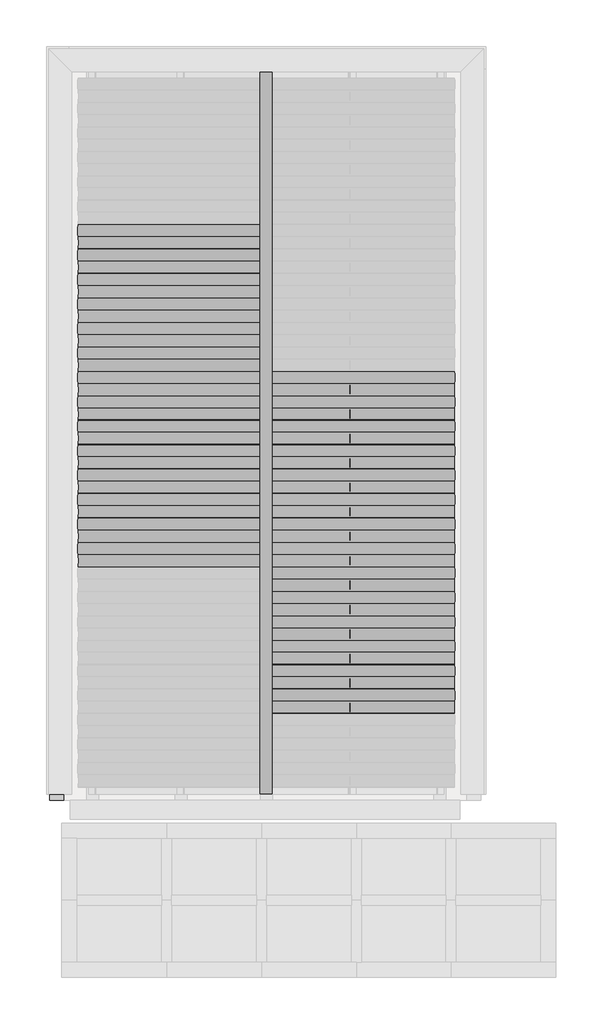
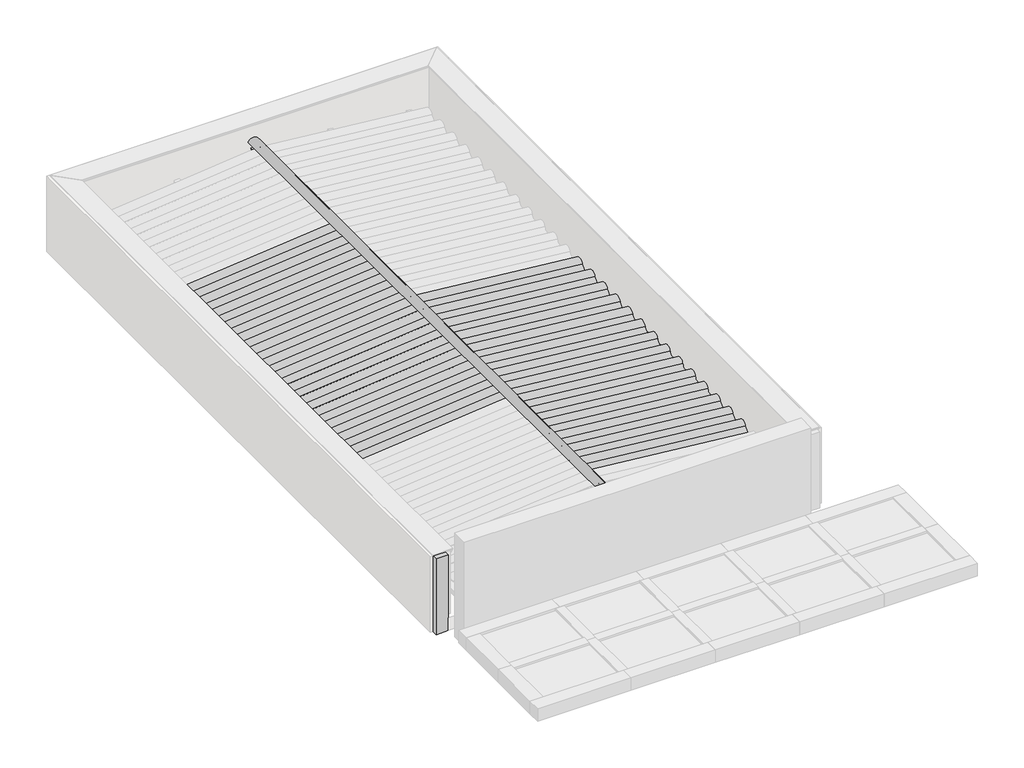
# One storey, part 2 of 3: 37 beams, 7 columns.
# Revit data of these elements (continued)
# Type "TQS - Viga retangular : 14.0 x 90.0" (continued)
#   h = 0.90 m
#   Structural Material [instance default] = none
#   Assembly Code = ""
# Type "Telha Ondulada : Fibrocimento"
#   Description = "TELHA ONDULADA FIBROCIMENTO"
#   Cost = 5
#   Length [instance default] = 1.524 m
#   b = 0.07 m
#   h = 0.16 m
#   Structural Material = .TELHA DE FIBROCIMENTO
#   Assembly Code = ""
# Type "Madeira de lei : Viga Cumeeira 6x16cm"
#   A = 0.02 m²
#   Length [instance default] = 1.524 m
#   b = 0.06 m
#   d = 0.16 m
#   Structural Material [instance default] = none
#   Assembly Code = ""
# Type "Madeira de lei-Coluna : Pontalete 6X16cm"
#   A = 0.01952 m²
#   b = 0.06 m
#   d = 0.16 m
#   Structural Material [instance default] = none
#   Assembly Code = ""
# Elements 1, 2, 3, 4, 5, 6 (IfcBeam, "Madeira de lei : Berço 6x12cm")
#   Comments = ""
#   Uso = "TELHADOS ESTRUTURAS"
#   Compr Cmcl = 6.00 m
#   Structural Material = .MADEIRAMENTO
#   Phase Created = CC_AP
#   Materials on its faces: ".MADEIRAMENTO"
# Element 7 (IfcBeam, "Cumeeira Telha Ondulada : Fibrocimento")
#   Comments = ""
#   Uso = "TELHADOS TELHAS"
#   Phase Created = CC_AP
#   Materials on its faces: ".TELHA DE FIBROCIMENTO"
# Element 8 (IfcBeam, "TQS - Viga retangular : 14.0 x 90.0")
#   Uso = "ESTRUTURA"
#   Titulo = "V103"
#   Chave = "-1269"
#   Tipo Elemento = "Viga"
#   SHA1 = "41485AF0083A76256DE091CB1906E367EBA2D647"
#   Revisão = ""
#   Tipo de carga = ""
#   Divisor de flexao = ""
#   Secao = ""
#   Configuracao = ""
#   Angulo (graus) = ""
#   Detalhamento = ""
#   Casos de vento manual = ""
#   Tipo = ""
#   Alcas = ""
#   Furos = ""
#   Pino = ""
#   Distribuicao = ""
#   Solidarizado = ""
#   Solidarizar na montagem = ""
#   Unir com o próximo = ""
#   Grupo pre moldado = ""
#   Verificado = ""
#   Concreto C = ""
#   Taxa de armadura (kgf/m³) = 0
#   Carga (tf/m²) = 0
#   Carga (tf/m) = 0
#   Carga (tf) = 0
#   Altura = 0.90 m
#   Rebaixo = -0.75 m
#   Largura = 0.14 m
#   Distancia a face = 0.00 m
#   Distancia ao eixo = 0.00 m
#   Altura gerber esquerda = 0.00 m
#   Largura gerber esquerda = 0.00 m
#   Altura gerber direita = 0.00 m
#   Largura gerber direita = 0.00 m
#   Resultado de Ensaios fck (MPa) = 0
#   Unique TQS ID = -1269
#   Principal = yes
#   Structural Material = none
#   Phase Created = CC_PE
# Elements 9, 10, 11, 12, 13, 14, 15, 16, 17, 18, 19, 20, 21, 22, 23, 24, 25, 26, 27, 28, 29, 30, 31, 32, 33, 34, 35, 36 (IfcBeam, "Telha Ondulada : Fibrocimento")
#   Uso = "TELHADOS TELHAS"
#   Phase Created = CC_AP
#   Materials on its faces: ".TELHA DE FIBROCIMENTO"
# Element 37 (IfcBeam, "Madeira de lei : Viga Cumeeira 6x16cm")
#   Comments = ""
#   Uso = "TELHADOS MADEIRAMENTO"
#   Compr Cmcl = 7.50 m
#   Structural Material = .MADEIRAMENTO
#   Phase Created = CC_AP
#   Materials on its faces: ".MADEIRAMENTO"
# Elements 38, 39, 40, 41, 42, 43, 44 (IfcColumn, "Madeira de lei-Coluna : Pontalete 6X16cm")
#   Comments = ""
#   Uso = "TELHADOS ESTRUTURAS"
#   Compr Cmcl = 2.00 m
#   Structural Material = .MADEIRAMENTO
#   Phase Created = CC_AP
#   Materials on its faces: ".MADEIRAMENTO"
# Materials
#   ".TELHA DE FIBROCIMENTO": class "CC_TELHADO", colour RGB 77 77 76, transparency 0, Description = "TELHA ONDULADA FIBROCIMENTO", Cost = 0
#   ".MADEIRAMENTO": class ".CC_MADEIRAS", colour RGB 212 179 113, transparency 0, Cost = 0
# Room, not placed, phase "CC_AP", upper offset 0.00 m, lower offset 0.00 m
#   Number = "31"
#   Name = "Room"
# Room, not placed, phase "CC_AP", upper offset 0.00 m, lower offset 0.00 m
#   Number = "34"
#   Name = "Room"
